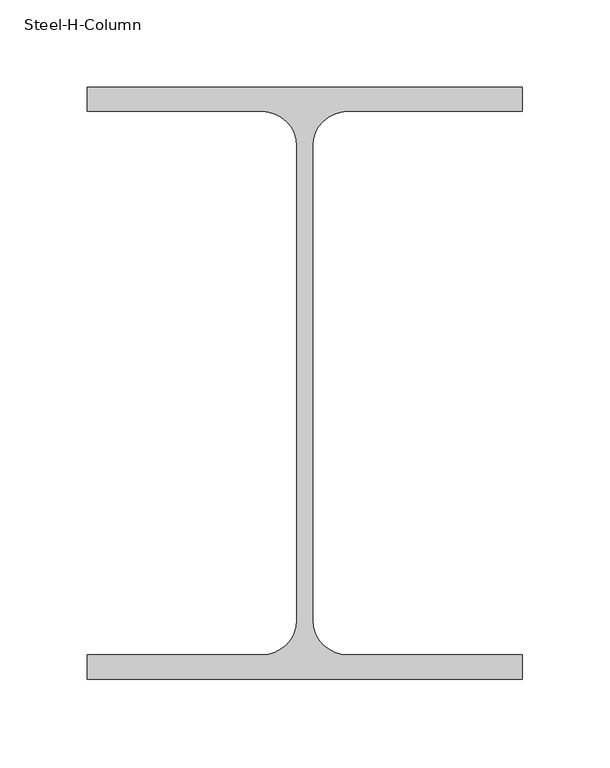
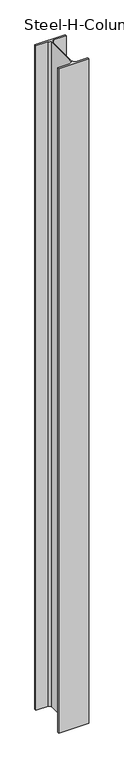
# IFC4 building model written with IfcOpenShell, lengths in millimetres: column geometry, Steel-H-Column : CL121_H-340×250x9x14.
# Revit data of these elements (continued)
# Project information (continued)
#     -cfd758078946\" /><element revit_id=\"af7cfdda-f71a-4a09-bb03-63e0c16d5d93-001530cf\" ism_id=\"46a5ded9-4fed-43a0-a06e-bb0fce603002\" /><element revit_id=\"af7cfdda-f71a-4a09-bb03-63e0c16d5d93-001530d1\" ism_id=\"62d05a0c-55f2-4c29-a355-b77f91c84c50\" /><element revit_id=\"af7cfdda-f71a-4a09-bb03-63e0c16d5d93-001530d3\" ism_id=\"eac0c420-7041-45a3-ad98-0cab4f5d8155\" /><element revit_id=\"af7cfdda-f71a-4a09-bb03-63e0c16d5d93-001530d5\" ism_id=\"9f5beb51-429a-4c7b-aa2e-ad2efe601ed6\" /><element revit_id=\"af7cfdda-f71a-4a09-bb03-63e0c16d5d93-001530d7\" ism_id=\"4613af3e-a189-4781-a937-106d789655c9\" /><element revit_id=\"af7cfdda-f71a-4a09-bb03-63e0c16d5d93-001530d9\" ism_id=\"71402e21-51c1-43b7-b8cc-75d2aba247eb\" /><element revit_id=\"af7cfdda-f71a-4a09-bb03-63e0c16d5d93-001530db\" ism_id=\"89101b83-9b84-4f11-b026-90cd564a3900\" /><element revit_id=\"af7cfdda-f71a-4a09-bb03-63e0c16d5d93-001530dd\" ism_id=\"37670781-ce23-4ce1-992b-7a400613c37b\" /><element revit_id=\"af7cfdda-f71a-4a09-bb03-63e0c16d5d93-001530df\" ism_id=\"2316856d-18eb-466b-8ab8-114816378db0\" /><element revit_id=\"af7cfdda-f71a-4a09-bb03-63e0c16d5d93-001530e2\" ism_id=\"da4f1597-5b5a-43a6-aa94-e478ffd6cfc7\" /><element revit_id=\"af7cfdda-f71a-4a09-bb03-63e0c16d5d93-001530e5\" ism_id=\"60805764-efb2-4434-8d81-aed3c3ed3c1b\" /><element revit_id=\"af7cfdda-f71a-4a09-bb03-63e0c16d5d93-001530e8\" ism_id=\"34e34ebb-6481-4bfb-b3d0-cb52295ff652\" /><element revit_id=\"af7cfdda-f71a-4a09-bb03-63e0c16d5d93-001530eb\" ism_id=\"dd5c4d73-1406-4c40-a955-5f9c52d01161\" /><element revit_id=\"af7cfdda-f71a-4a09-bb03-63e0c16d5d93-001530ed\" ism_id=\"cf8abc6b-638f-4bd5-8b66-615be032e220\" /><element revit_id=\"af7cfdda-f71a-4a09-bb03-63e0c16d5d93-001530f0\" ism_id=\"56ce8857-0c24-48d5-82f2-459e263998e2\" /><element revit_id=\"af7cfdda-f71a-4a09-bb03-63e0c16d5d93-001530f2\" ism_id=\"a1f000e8-ea08-442b-8a96-da7657653fd5\" /><element revit_id=\"af7cfdda-f71a-4a09-bb03-63e0c16d5d93-001530f4\" ism_id=\"2625e954-f7fb-41eb-b9bd-1b615ef945fc\" /><element revit_id=\"af7cfdda-f71a-4a09-bb03-63e0c16d5d93-001530f6\" ism_id=\"48469362-393c-4deb-bbb2-ad00180a23fb\" /><element revit_id=\"af7cfdda-f71a-4a09-bb03-63e0c16d5d93-001530f8\" ism_id=\"8e650f6f-0906-45a9-8fb8-35680155d6db\" /><element revit_id=\"af7cfdda-f71a-4a09-bb03-63e0c16d5d93-001530fb\" ism_id=\"f84acaf6-20a1-4df6-afed-1dc07fd0b2e9\" /><element revit_id=\"af7cfdda-f71a-4a09-bb03-63e0c16d5d93-001530fe\" ism_id=\"72816c7e-9128-47f4-b46a-ee567a2a03d6\" /><element revit_id=\"af7cfdda-f71a-4a09-bb03-63e0c16d5d93-00153100\" ism_id=\"c95ab0f8-b4bf-4b7c-bd1d-0423c8ac725a\" /><element revit_id=\"af7cfdda-f71a-4a09-bb03-63e0c16d5d93-00153102\" ism_id=\"32fd4119-6673-4973-aef2-b39ef90310e5\" /><element revit_id=\"af7cfdda-f71a-4a09-bb03-63e0c16d5d93-00153104\" ism_id=\"fd2aa4a6-d123-4100-85b9-db27c20cf6bc\" /><element revit_id=\"af7cfdda-f71a-4a09-bb03-63e0c16d5d93-00153106\" ism_id=\"e00fdefa-e77c-4406-9dbe-3c9122259821\" /><element revit_id=\"af7cfdda-f71a-4a09-bb03-63e0c16d5d93-00153108\" ism_id=\"25e5b79e-07c2-4ffa-a7a9-bf039dd2ad78\" /><element revit_id=\"af7cfdda-f71a-4a09-bb03-63e0c16d5d93-0015310b\" ism_id=\"720021d4-ca74-47c0-9c64-7d0854fa39f5\" /><element revit_id=\"af7cfdda-f71a-4a09-bb03-63e0c16d5d93-0015310d\" ism_id=\"ea922120-0cff-4f8d-a5c2-2841c031873e\" /><element revit_id=\"af7cfdda-f71a-4a09-bb03-63e0c16d5d93-0015310f\" ism_id=\"9d07ca73-3a65-44fe-ab61-476d8d1352d1\" /><element revit_id=\"af7cfdda-f71a-4a09-bb03-63e0c16d5d93-00153111\" ism_id=\"68a2fb30-d213-40c7-a166-dad5a20bd269\" /><element revit_id=\"af7cfdda-f71a-4a09-bb03-63e0c16d5d93-00153113\" ism_id=\"06119775-28f9-44f0-a265-5c57029016d1\" /><element revit_id=\"af7cfdda-f71a-4a09-bb03-63e0c16d5d93-00153115\" ism_id=\"ca133383-8253-4d07-aa92-f507fbb2ee47\" /><element revit_id=\"af7cfdda-f71a-4a09-bb03-63e0c16d5d93-00153117\" ism_id=\"6f4a7c07-4bd3-4c99-b1e4-110c964ccc07\" /><element revit_id=\"af7cfdda-f71a-4a09-bb03-63e0c16d5d93-00153119\" ism_id=\"ee1f865b-98a9-4ff1-a84c-52926e8f3566\" /><element revit_id=\"af7cfdda-f71a-4a09-bb03-63e0c16d5d93-0015311b\" ism_id=\"4fd7bd5c-7c46-4e79-a72b-dab4a1d98f33\" /><element revit_id=\"af7cfdda-f71a-4a09-bb03-63e0c16d5d93-0015311e\" ism_id=\"9ca0cac6-aaff-412a-b9c1-a8be985bc44a\" /><element revit_id=\"af7cfdda-f71a-4a09-bb03-63e0c16d5d93-00153121\" ism_id=\"73123639-76b5-46f0-a49e-b26af36d93b1\" /><element revit_id=\"af7cfdda-f71a-4a09-bb03-63e0c16d5d93-00153123\" ism_id=\"f74e8cb9-a93d-4aaa-985b-c0ed9befad19\" /><element revit_id=\"af7cfdda-f71a-4a09-bb03-63e0c16d5d93-00153126\" ism_id=\"5778daa1-b4cb-4cc3-9b7d-323562a47fba\" /><element revit_id=\"af7cfdda-f71a-4a09-bb03-63e0c16d5d93-00153129\" ism_id=\"2d7457d2-8978-4c95-9056-ebbaed3263eb\" /><element revit_id=\"af7cfdda-f71a-4a09-bb03-63e0c16d5d93-0015312c\" ism_id=\"48b420ce-6767-430a-aadc-695c25361a2d\" /><element revit_id=\"af7cfdda-f71a-4a09-bb03-63e0c16d5d93-0015312e\" ism_id=\"fc34038c-136d-4d55-b951-9cc35899fd33\" /><element revit_id=\"af7cfdda-f71a-4a09-bb03-63e0c16d5d93-00153130\" ism_id=\"e7a25938-3b91-4519-a48d-86fdd79489d5\" /><element revit_id=\"af7cfdda-f71a-4a09-bb03-63e0c16d5d93-00153133\" ism_id=\"c81dfd8c-579c-4d77-ab89-bf1f415d9cc6\" /><element revit_id=\"af7cfdda-f71a-4a09-bb03-63e0c16d5d93-00153136\" ism_id=\"5756a4b4-84ca-418c-b9f6-2d2370afca2f\" /><element revit_id=\"af7cfdda-f71a-4a09-bb03-63e0c16d5d93-0015313a\" ism_id=\"09a9cede-a757-4d8e-a722-6140af98bc61\" /><element revit_id=\"af7cfdda-f71a-4a09-bb03-63e0c16d5d93-0015313d\" ism_id=\"ac9b583c-7f63-4351-8b69-3967279b234c\" /><element revit_id=\"af7cfdda-f71a-4a09-bb03-63e0c16d5d93-00153140\" ism_id=\"1a52584d-6b21-4de6-bb42-5b9bdd6f24e9\" /><element revit_id=\"af7cfdda-f71a-4a09-bb03-63e0c16d5d93-00153143\" ism_id=\"6c2e2bc0-8432-4c98-9292-cbb2182bd4b0\" /><element revit_id=\"af7cfdda-f71a-4a09-bb03-63e0c16d5d93-00153145\" ism_id=\"644bb900-7654-42c5-a9b7-996a2197f6d0\" /><element revit_id=\"af7cfdda-f71a-4a09-bb03-63e0c16d5d93-00153148\" ism_id=\"a1bca0bd-75db-464c-b27a-2a69d9b4ad3d\" /><element revit_id=\"af7cfdda-f71a-4a09-bb03-63e0c16d5d93-0015314a\" ism_id=\"ea29955b-34f2-409a-aefa-e6adfe75349e\" /><element revit_id=\"af7cfdda-f71a-4a09-bb03-63e0c16d5d93-0015314d\" ism_id=\"800fef33-e5e1-422c-b708-e9394bbeefcc\" /><element revit_id=\"af7cfdda-f71a-4a09-bb03-63e0c16d5d93-0015314f\" ism_id=\"86259dca-8773-4253-ac56-e71252267c8a\" /><element revit_id=\"af7cfdda-f71a-4a09-bb03-63e0c16d5d93-00153152\" ism_id=\"d15a0ad2-db9f-420d-bea3-41a78a0eb330\" /><element revit_id=\"af7cfdda-f71a-4a09-bb03-63e0c16d5d93-00153155\" ism_id=\"bd27f420-df49-4abe-bd96-8e48e7f4efcb\" /><element revit_id=\"af7cfdda-f71a-4a09-bb03-63e0c16d5d93-00153157\" ism_id=\"5d451f94-860d-4cc3-a4fa-51a9f3126e33\" /><element revit_id=\"af7cfdda-f71a-4a09-bb03-63e0c16d5d93-0015315a\" ism_id=\"4234158a-994a-492b-85da-6108709b7232\" /><element revit_id=\"af7cfdda-f71a-4a09-bb03-63e0c16d5d93-0015315c\" ism_id=\"ca24c92d-986b-417f-812f-024ab15e24c8\" /><element revit_id=\"af7cfdda-f71a-4a09-bb03-63e0c16d5d93-0015315f\" ism_id=\"699ec3b0-0151-4110-b054-14418651f324\" /><element revit_id=\"af7cfdda-f71a-4a09-bb03-63e0c16d5d93-00153161\" ism_id=\"38ecdeac-3d85-48dd-82c1-53fe93f49beb\" /><element revit_id=\"af7cfdda-f71a-4a09-bb03-63e0c16d5d93-00153163\" ism_id=\"1340aefd-b79c-4264-8a49-d0a0504eff8c\" /><element revit_id=\"af7cfdda-f71a-4a09-bb03-63e0c16d5d93-00153165\" ism_id=\"1b6167c2-fb26-4b8d-916b-d835d89896e7\" /><element revit_id=\"af7cfdda-f71a-4a09-bb03-63e0c16d5d93-00153167\" ism_id=\"290d3d83-57eb-4125-aecb-a977a5fcf5ca\" /><element revit_id=\"af7cfdda-f71a-4a09-bb03-63e0c16d5d93-00153169\" ism_id=\"105c9b97-1c70-4237-82ac-8404a3e8e6a6\" /><element revit_id=\"af7cfdda-f71a-4a09-bb03-63e0c16d5d93-0015316c\" ism_id=\"1726c5bb-05e2-4959-9da2-4227f0219f00\" /><element revit_id=\"af7cfdda-f71a-4a09-bb03-63e0c16d5d93-0015316e\" ism_id=\"d919ee9c-caed-4119-b451-e3644db952c8\" /><element revit_id=\"af7cfdda-f71a-4a09-bb03-63e0c16d5d93-00153170\" ism_id=\"1b1fab26-60c4-40ed-b31b-b177eda246ce\" /><element revit_id=\"af7cfdda-f71a-4a09-bb03-63e0c16d5d93-00153172\" ism_id=\"ea9b5221-a1f2-4796-8cca-f7872ab69cbd\" /><element revit_id=\"af7cfdda-f71a-4a09-bb03-63e0c16d5d93-00153174\" ism_id=\"660b40b2-06fb-4b62-b987-28a171e473fe\" /><element revit_id=\"af7cfdda-f71a-4a09-bb03-63e0c16d5d93-00153176\" ism_id=\"767be0d9-c5ba-4ad3-a52d-efd60031fc9a\" /><element revit_id=\"af7cfdda-f71a-4a09-bb03-63e0c16d5d93-00153178\" ism_id=\"6fbe93ce-4ed7-4596-88fc-71dafe48803e\" /><element revit_id=\"af7cfdda-f71a-4a09-bb03-63e0c16d5d93-0015317a\" ism_id=\"27d7b093-4eb7-47aa-b123-5388a6327d7f\" /><element revit_id=\"af7cfdda-f71a-4a09-bb03-63e0c16d5d93-0015317c\" ism_id=\"9073a947-5952-42fe-b37a-cdfed3ca30c7\" /><element revit_id=\"af7cfdda-f71a-4a09-bb03-63e0c16d5d93-0015317e\" ism_id=\"1888f060-aa3c-4494-8f30-a80ca2311216\" /><element revit_id=\"af7cfdda-f71a-4a09-bb03-63e0c16d5d93-00153181\" ism_id=\"c0491dc2-5df2-4c14-b988-e117f6f511a2\" /><element revit_id=\"af7cfdda-f71a-4a09-bb03-63e0c16d5d93-00153184\" ism_id=\"4f44b9aa-c092-46fe-bf9b-2d1be872d419\" /><element revit_id=\"af7cfdda-f71a-4a09-bb03-63e0c16d5d93-00153186\" ism_id=\"eb560801-76cf-40a8-a181-31cd32aca14f\" /><element revit_id=\"af7cfdda-f71a-4a09-bb03-63e0c16d5d93-00153189\" ism_id=\"8d1e5f00-41d5-42c1-9b4f-a8c2eb689a72\" /><element revit_id=\"af7cfdda-f71a-4a09-bb03-63e0c16d5d93-0015318b\" ism_id=\"caf6c2dc-0e9e-46a9-a3e1-71316081ff61\" /><element revit_id=\"af7cfdda-f71a-4a09-bb03-63e0c16d5d93-0015318d\" ism_id=\"4d149f88-f5b9-4943-8765-090324e0a65d\" /><element revit_id=\"af7cfdda-f71a-4a09-bb03-63e0c16d5d93-0015318f\" ism_id=\"75865cf2-3adc-4a52-a778-fc6fb65fcdcb\" /><element revit_id=\"af7cfdda-f71a-4a09-bb03-63e0c16d5d93-00153191\" ism_id=\"f9320017-2083-48f1-8aff-e6ba958fb1c5\" /><element revit_id=\"af7cfdda-f71a-4a09-bb03-63e0c16d5d93-00153193\" ism_id=\"38a61c12-98f2-47b1-843d-8351040e24d2\" /><element revit_id=\"af7cfdda-f71a-4a09-bb03-63e0c16d5d93-00153196\" ism_id=\"af709a9c-b664-480b-be0d-fb01aac630f2\" /><element revit_id=\"af7cfdda-f71a-4a09-bb03-63e0c16d5d93-00153199\" ism_id=\"a4c2867c-ca2a-4112-b86c-4e6563e3dc63\" /><element revit_id=\"14a48413-84c4-4e00-9e64-4f618415469a-0013ce74\" ism_id=\"F2ADF140-E21A-4820-8170-6F63D956DCAD\" /><element revit_id=\"14a48413-84c4-4e00-9e64-4f618415469a-0013ce74\" ism_id=\"B35A310E-4F33-462b-819C-3ADD300C0CEB\" /><element revit_id=\"14a48413-84c4-4e00-9e64-4f618415469a-0013ce74\" ism_id=\"711054EC-0DB2-46e3-AD20-004560300C00\" /><element revit_id=\"14a48413-84c4-4e00-9e64-4f618415469a-0013ce6e\" ism_id=\"B5C54EC9-8EBD-4860-AB72-EF5791AED394\" /><element revit_id=\"14a48413-84c4-4e00-9e64-4f618415469a-0013e793\" ism_id=\"0A7B8D02-9EA4-4aa9-A41A-E30BB5B6B6C5\" /><element revit_id=\"14a48413-84c4-4e00-9e64-4f618415469a-0013e793\" ism_id=\"714BBD27-DB58-47da-B54C-5806291C2D3C\" /><element revit_id=\"14a48413-84c4-4e00-9e64-4f618415469a-0013e793\" ism_id=\"F36E62C1-13EE-4807-A3C1-899E23E0BEDE\" /><element revit_id=\"14a48413-84c4-4e00-9e64-4f618415469a-0013e793\" ism_id=\"F5448801-679E-44d6-8F46-E676344F8165\" /><element revit_id=\"14a48413-84c4-4e00-9e64-4f618415469a-0013e793\" ism_id=\"846DCB0C-E06B-4978-9D43-E1CC0FDE7595\" /><element revit_id=\"14a48413-84c4-4e00-9e64-4f618415469a-0013e793\" ism_id=\"2ADF82B8-986D-4f44-85DE-89D921292160\" /><element revit_id=\"14a48413-84c4-4e00-9e64-4f618415469a-0013e793\" ism_id=\"7AF371ED-051B-4a30-8826-11F11C212B73\" /><element revit_id=\"14a48413-84c4-4e00-9e64-4f618415469a-0013e793\" ism_id=\"2FE74006-ADDA-412f-A522-853919E62B4D\" /><element revit_id=\"14a48413-84c4-4e00-9e64-4f618415469a-0013e793\" ism_id=\"09B63641-D581-4a6c-A18E-54C17EC989A4\" /><element revit_id=\"14a48413-84c4-4e00-9e64-4f618415469a-0013e793\" ism_id=\"0DD6B52A-77D0-45a1-82B1-8236ED57078C\" /><element revit_id=\"14a48413-84c4-4e00-9e64-4f618415469a-0013e793\" ism_id=\"35D311D2-DEB8-4469-97DE-110B6DF5B84D\" /><element revit_id=\"14a48413-84c4-4e00-9e64-4f618415469a-0013e79
#     3\" ism_id=\"0D3CCDE5-CFF9-431b-A4BD-01BF6636D6BD\" /><element revit_id=\"14a48413-84c4-4e00-9e64-4f618415469a-0013e793\" ism_id=\"C62B2A5B-024A-47ac-B030-C17A67E64A7B\" /><element revit_id=\"14a48413-84c4-4e00-9e64-4f618415469a-0013e793\" ism_id=\"944C6E43-E607-48c3-8358-9E6CB88346E7\" /><element revit_id=\"14a48413-84c4-4e00-9e64-4f618415469a-0013e793\" ism_id=\"A4B1F42D-B1C2-4ad2-8AD6-DB0D5E05998D\" /><element revit_id=\"14a48413-84c4-4e00-9e64-4f618415469a-0013e793\" ism_id=\"007E6C70-1139-4b48-B003-C76FAD4C249A\" /><element revit_id=\"14a48413-84c4-4e00-9e64-4f618415469a-0013e793\" ism_id=\"9941AC94-F03A-464c-9912-04590E0C31E0\" /><element revit_id=\"14a48413-84c4-4e00-9e64-4f618415469a-0013e793\" ism_id=\"CFD98B8D-8FF4-4e71-A909-0FE7DBCE924E\" /><element revit_id=\"14a48413-84c4-4e00-9e64-4f618415469a-0013e793\" ism_id=\"58262161-98E6-45c8-B2BD-4508105FF662\" /><element revit_id=\"14a48413-84c4-4e00-9e64-4f618415469a-0013e793\" ism_id=\"66AB4841-610A-4883-97F7-1282A56484E1\" /><element revit_id=\"14a48413-84c4-4e00-9e64-4f618415469a-0013e793\" ism_id=\"D2B324BE-BBD6-49da-9730-60EA7AD4D3A0\" /><element revit_id=\"14a48413-84c4-4e00-9e64-4f618415469a-0013e793\" ism_id=\"92A8ECE7-C053-46b1-92ED-F2C041617E7B\" /><element revit_id=\"14a48413-84c4-4e00-9e64-4f618415469a-0013e793\" ism_id=\"B4C4BDB0-65C4-4016-9C78-DBD77E229523\" /><element revit_id=\"14a48413-84c4-4e00-9e64-4f618415469a-0013e793\" ism_id=\"57270646-162F-4c83-BDB7-A5FBEA9120BD\" /><element revit_id=\"14a48413-84c4-4e00-9e64-4f618415469a-0013e793\" ism_id=\"BDEF733F-00AA-4eee-B6C6-50229FC1D236\" /><element revit_id=\"14a48413-84c4-4e00-9e64-4f618415469a-0013e793\" ism_id=\"84A94E1E-3074-40f4-9690-97191755F019\" /><element revit_id=\"14a48413-84c4-4e00-9e64-4f618415469a-0013e793\" ism_id=\"8A7D913D-7967-4718-912D-B83DF0AD2EDD\" /><element revit_id=\"14a48413-84c4-4e00-9e64-4f618415469a-0013e793\" ism_id=\"83553D70-90FA-469c-B5C3-EF03F3FC6475\" /><element revit_id=\"14a48413-84c4-4e00-9e64-4f618415469a-0013e793\" ism_id=\"6880C1E4-C50B-4c1b-B61C-23F2D8C46873\" /><element revit_id=\"14a48413-84c4-4e00-9e64-4f618415469a-0013e793\" ism_id=\"08594C43-CD40-47de-A3BA-8BFB47F64994\" /><element revit_id=\"14a48413-84c4-4e00-9e64-4f618415469a-0013e793\" ism_id=\"7D2E11FA-A5E1-4434-B9BE-AABA1A16CA03\" /><element revit_id=\"14a48413-84c4-4e00-9e64-4f618415469a-0013e793\" ism_id=\"D892DFA4-5441-4ad2-A390-253492293B1B\" /><element revit_id=\"14a48413-84c4-4e00-9e64-4f618415469a-0013e793\" ism_id=\"E5A32FE6-89C4-49f1-B3B9-1CABE7C48A4D\" /><element revit_id=\"14a48413-84c4-4e00-9e64-4f618415469a-0013e793\" ism_id=\"8AE872C2-5DBE-47c5-934B-7E964A84B589\" /><element revit_id=\"14a48413-84c4-4e00-9e64-4f618415469a-0013e793\" ism_id=\"3C847B60-488A-4604-A400-16A3A65E919B\" /><element revit_id=\"14a48413-84c4-4e00-9e64-4f618415469a-0013e793\" ism_id=\"DBEC432A-3F7B-4266-AD99-2A937DC70BCF\" /><element revit_id=\"14a48413-84c4-4e00-9e64-4f618415469a-0013e793\" ism_id=\"59403DD6-7A51-48aa-A3BE-962457E6F10E\" /><element revit_id=\"14a48413-84c4-4e00-9e64-4f618415469a-0013e793\" ism_id=\"11CDDF5D-38B6-43b2-A291-FC188BE232BC\" /><element revit_id=\"14a48413-84c4-4e00-9e64-4f618415469a-0013e793\" ism_id=\"10BF2843-EFC9-4136-933C-5B270D970277\" /><element revit_id=\"14a48413-84c4-4e00-9e64-4f618415469a-0013e793\" ism_id=\"E1B09A9C-F6C6-47d9-976B-E313C0E3F52B\" /><element revit_id=\"14a48413-84c4-4e00-9e64-4f618415469a-0013e793\" ism_id=\"A3A22EC3-26C8-4588-A0AB-AFAE02DF267E\" /><element revit_id=\"14a48413-84c4-4e00-9e64-4f618415469a-0013e793\" ism_id=\"114828FC-BDC1-4343-9119-BCB5395DAA64\" /><element revit_id=\"14a48413-84c4-4e00-9e64-4f618415469a-0013e793\" ism_id=\"797626F9-3558-4623-826F-15FB93088CB3\" /><element revit_id=\"14a48413-84c4-4e00-9e64-4f618415469a-0013e793\" ism_id=\"4BF369CD-DF09-4346-96CB-C6C6380A2599\" /><element revit_id=\"14a48413-84c4-4e00-9e64-4f618415469a-0013e793\" ism_id=\"722B46BA-61C4-44a1-9ECF-325B60B6688D\" /><element revit_id=\"14a48413-84c4-4e00-9e64-4f618415469a-0013e793\" ism_id=\"C33DBE84-19C1-4379-AB6E-A41F7420F18C\" /><element revit_id=\"14a48413-84c4-4e00-9e64-4f618415469a-0013e793\" ism_id=\"1F2D3B75-66F2-4d88-A1DD-647969477B86\" /><element revit_id=\"14a48413-84c4-4e00-9e64-4f618415469a-0013e793\" ism_id=\"DFBF96B2-410A-4f39-80C4-D8CF78561C93\" /><element revit_id=\"14a48413-84c4-4e00-9e64-4f618415469a-0013e793\" ism_id=\"D6793CD3-AB64-417c-9C28-8B18A0A2D336\" /><element revit_id=\"14a48413-84c4-4e00-9e64-4f618415469a-0013e793\" ism_id=\"90884AC0-EA00-4caa-86E1-E6B886FD90ED\" /><element revit_id=\"14a48413-84c4-4e00-9e64-4f618415469a-0013e793\" ism_id=\"64BC7B89-F7C8-4dae-A5C8-F10DF9E5F6BA\" /><element revit_id=\"14a48413-84c4-4e00-9e64-4f618415469a-0013e793\" ism_id=\"D82E4D85-2728-40e5-9F60-1C7FB2990D78\" /><element revit_id=\"14a48413-84c4-4e00-9e64-4f618415469a-0013e793\" ism_id=\"1E6D05B9-BF84-4669-AA27-948ADA1D511E\" /><element revit_id=\"14a48413-84c4-4e00-9e64-4f618415469a-0013e793\" ism_id=\"73608CB2-EB94-466e-883D-814030EF49D6\" /><element revit_id=\"14a48413-84c4-4e00-9e64-4f618415469a-0013e793\" ism_id=\"4EAF07EF-4E08-4065-9F08-BF69D4413867\" /><element revit_id=\"14a48413-84c4-4e00-9e64-4f618415469a-0013e0e9\" ism_id=\"05D74241-6318-4cac-95F5-7B878260D5B5\" /></element_binding><reinforcement_properties /><operation_settings><coordinate_mapping x=\"0\" y=\"0\" z=\"0\" /></operation_settings></ism>"
#   Building Name = "FIRE WATER PUMP BUILDING"
#   Project Status = "Project Status"
#   Client Name = "현대엔지니어링"
#   Project Address = "서울시 종로구 율곡로 75(계동)"
#   Project Name = "TAKHIATASH POWER PLANT EFFICIENCY IMPROVEMENT PROJECT / 우즈베키스탄"
#   Project Number = "BEUZ1602"
#   F01) Building Name = "FIRE WATER PUMP BUILDING"
#   F11) Project Building Tag_Type-1 = "BI aWBS"
#   F12) Project Building Tag_Type-2 = "BI aWBS"
#   F13) Project Facility Code = "621"
#   F21) Structural Type = "STEEL"
#   F31) Standard Building Code = "E204"
#   F41) Discipline = "Architecture"
#   F51) Plan Start Date-Engineering = "2018-01-01"
#   F52) Plan Finish Date-Engineering = "2018-09-13"
#   F53) Duration = "255"
#   F61) Plan Start Date-Construction = "2018-09-14"
#   F62) Plan Finish Date-Construction = "2019-12-02"
#   F63) Duration = "444"
#   F91) Plant Type = "2GTG+2STG+1HRSG"
#   F92) KKS Structures, Building = "UAB"
#   P01) Project Name = "TAKHIATASH POWER PLANT EFFICIENCY IMPROVEMENT PROJECT / 우즈베키스탄"
#   P02) Project Configuration = "2 GTG + 2 HRSG + 2STG, 2 x 250MW"
#   P03) Project Abbreviation = "UTCC"
#   P04) Project Code = "BEUZ1602"
#   P05) Project Stage = "실행"
#   P06) Project Location = "Takhiatash / Uzbekistan"
#   P07) Project Owner = "우즈베키스탄 전력청"
#   P08) Project O.E = "GAS Natural Fenosa"
#   P09) Project Schedule = "2017.10.01 ~ 2020.08.08"
#   P10) Basic Wind Speed = "48m/sec_ASCE7-05"
#   P11) Seismic = "SDS_0.15_ASCE7-05"
#   P12) Soil = "SD_ASCE7-05"
#   P13) Soil Capacity = "400 kN/m2_Soil Replacement"
#   P14) Pile Capacity = "1000 kN_D600 Board Pile"
# Type "Steel-H-Column : CL121_H-340×250x9x14"
#   Surface Area = 0.00 m²/m
#   Section Area = 101.5 cm²
#   Mass per Unit Length = 79.70 kg/m
#   B = 250 mm
#   H = 340 mm
#   r = 20 mm
#   tw = 9 mm
#   tf = 14 mm
#   hec_material4 [instance default] = none
#   hec_material2 [instance default] = none
#   hec_material1 [instance default] = none
#   hec_material3 [instance default] = none
#   Structural Material [instance default] = Steel, 45-345
#   Assembly Code = ""
# Element 1 (IfcColumn, "Steel-H-Column : CL121_H-340×250x9x14")
#   hec_material1 = S03AA028-00001_Main Steel Structure Erection Work_Shelter/Building_Medium Steel
#   hec_material3 = F01AC000-00002_Building/Shelter Fire Proofing Work_Intumescent Coating Type_1 hr. rating (UL 1709))
#   Structural Material = S01AA002-00001_Main Steel Structure Fabrication Work_Shelter/Building_Medium Steel - Standard
#   Materials on its faces: "S01AA002-00001_Main Steel Structure Fabrication Work_Shelter/Building_Medium Steel - Standard"
# Materials
#   "Steel, 45-345": class "Metal", colour RGB 189 187 185, transparency 0, Description = "Steel 345 MPa", Cost = 0
#   "S01AA002-00001_Main Steel Structure Fabrication Work_Shelter/Building_Medium Steel - Standard": class "Metal", colour RGB 120 120 120, transparency 0, Comments = "(90KG/M>Weight≥30KG/M)", Description = "Structural steel 50ksi", W00) Work Master Code = "S01AA002-0001", W01) Work Master_Lv1 = "Main Steel Structure Fabrication Work", W02) Work Master_Lv2 = "Shelter/Building", W03) Work Master_Spec.1 = "Medium Steel - Standard (90KG/M>Weight≥30KG/M)", Cost = 0
#   "S03AA028-00001_Main Steel Structure Erection Work_Shelter/Building_Medium Steel": class "Metal", colour RGB 120 120 120, transparency 0, Comments = "(90KG/M>Weight≥30KG/M)", Description = "Structural steel 50ksi", W00) Work Master Code = "S03AA028-0001", W01) Work Master_Lv1 = "Main Steel Structure Erection Work", W02) Work Master_Lv2 = "Shelter/Building", W03) Work Master_Spec.1 = "Medium Steel (90KG/M>Weight≥30KG/M)", Cost = 0
#   "F01AC000-00002_Building/Shelter Fire Proofing Work_Intumescent Coating Type_1 hr. rating (UL 1709))": class "Metal", colour RGB 255 128 128, transparency 0, Description = "Paint finished steel", W00) Work Master Code = "F01AC000-00002", W01) Work Master_Lv1 = "Building/Shelter Fire Proofing Work", W02) Work Master_Lv2 = "Intumescent Coating Type", W03) Work Master_Spec.1 = "1 hr. rating (UL 1709)", Cost = 0
